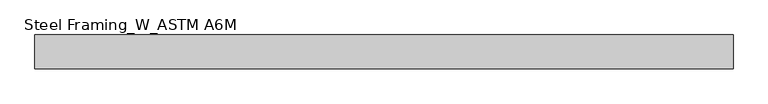
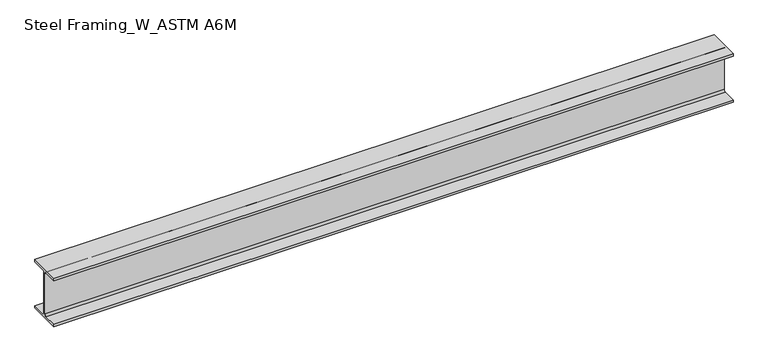
"""IFC4 building model written with IfcOpenShell, lengths in millimetres: beam geometry, Steel Framing_W_ASTM A6M : H_SB_AR_S02_W200x31.3_B6."""

from ifc_helpers import new_model, si_unit, point, frame, frame_2d, origin, place, context, project, spatial, polyline, circle_curve, trimmed, segment, composite_curve, outline, extrude, source, transform, mapped, element, save


def steel_framing_w_astm_a6m_fe1e75f4(model_context):
    return source(origin(), model_context, "Body", "SweptSolid", [
        extrude(outline(composite_curve([segment(polyline([(67.0, -94.8), (67.0, -105.0), (-67.0, -105.0), (-67.0, -94.8), (-10.775, -94.8)]), True, "CONTINUOUS"), segment(trimmed(circle_curve(frame_2d((-10.775, -87.2)), 7.6), [point((-10.775, -94.8))], [point((-3.175, -87.2))], True, "CARTESIAN"), True, "CONTINUOUS"), segment(polyline([(-3.175, -87.2), (-3.175, 87.2)]), True, "CONTINUOUS"), segment(trimmed(circle_curve(frame_2d((-10.775, 87.2)), 7.6), [point((-3.175, 87.2))], [point((-10.775, 94.8))], True, "CARTESIAN"), True, "CONTINUOUS"), segment(polyline([(-10.775, 94.8), (-67.0, 94.8), (-67.0, 105.0), (67.0, 105.0), (67.0, 94.8), (10.775, 94.8)]), True, "CONTINUOUS"), segment(trimmed(circle_curve(frame_2d((10.775, 87.2)), 7.6), [point((10.775, 94.8))], [point((3.175, 87.2))], True, "CARTESIAN"), True, "CONTINUOUS"), segment(polyline([(3.175, 87.2), (3.175, -87.2)]), True, "CONTINUOUS"), segment(trimmed(circle_curve(frame_2d((10.775, -87.2)), 7.6), [point((3.175, -87.2))], [point((10.775, -94.8))], True, "CARTESIAN"), True, "CONTINUOUS"), segment(polyline([(10.775, -94.8), (67.0, -94.8)]), True, "CONTINUOUS")], self_intersect=False)), frame((-1386.3, 0.0, 0.0), z_axis=(1.0, 0.0, 0.0), x_axis=(0.0, 1.0, 0.0)), (0.0, 0.0, 1.0), 2772.6),
    ])


if __name__ == "__main__":
    model = new_model("IFC4")
    model_context = context("Model", 3, world=origin())
    ifc_project = project(units=[si_unit("LENGTHUNIT", "METRE", prefix="MILLI")], contexts=[model_context])
    site = spatial("IfcSite", under=ifc_project)
    building = spatial("IfcBuilding", under=site)
    placement = place(None, origin())
    steel_framing_w_astm_a6m_shape = steel_framing_w_astm_a6m_fe1e75f4(model_context)
    element("IfcBeam", 1, ObjectType="Steel Framing_W_ASTM A6M : H_SB_AR_S02_W200x31.3_B6", at=placement, inside=building, context=model_context, shape_type="MappedRepresentation", body=[
        mapped(steel_framing_w_astm_a6m_shape, transform((0.0, 0.0, 0.0), x_axis=(1.0, 0.0, 0.0), y_axis=(0.0, 1.0, 0.0), z_axis=(0.0, 0.0, 1.0))),
    ])
    save(model, "model.ifc")

# Revit data of these elements
# Type "Steel Framing_W_ASTM A6M : H_SB_AR_S02_W200x31.3_B6"
#   Type Mark = "B6"
#   Section Name Key = "W8x21"
#   Width = 13.4 cm
#   Web Thickness = 0.635 cm
#   Web Fillet = 0.76 cm
#   Warping Constant = 40800.0 cm⁶
#   Torsional Moment of Inertia = 11.70 cm⁴
#   Section Area = 39.7 cm²
#   Plastic Modulus weak axis = 93.2 cm³
#   Plastic Modulus strong axis = 334.0 cm³
#   Perimeter = 0.93 m²/m
#   Nominal Weight = 31.30 kgf/m
#   Moment of Inertia weak axis = 407.00 cm⁴
#   Moment of Inertia strong axis = 3130.00 cm⁴
#   Height = 21.0 cm
#   Flange Thickness = 1.02 cm
#   Elastic Modulus weak axis = 60.8 cm³
#   Elastic Modulus strong axis = 298.0 cm³
#   Centroid Vertical = 10.5 cm
#   Centroid Horizontal = 6.7 cm
#   Length [instance default] = 1500 mm
#   Structural Material [instance default] = Steel, 45-345
#   Bolt Spacing = 0
#   Assembly Code = ""
# Element 1 (IfcBeam, "Steel Framing_W_ASTM A6M : H_SB_AR_S02_W200x31.3_B6")
#   Materials on its faces: "Steel, 45-345"
# Materials
#   "Steel, 45-345": class "Metal", colour RGB 189 187 185, transparency 0, Description = "Steel 345 MPa", Cost = 0
